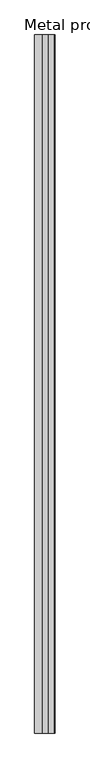
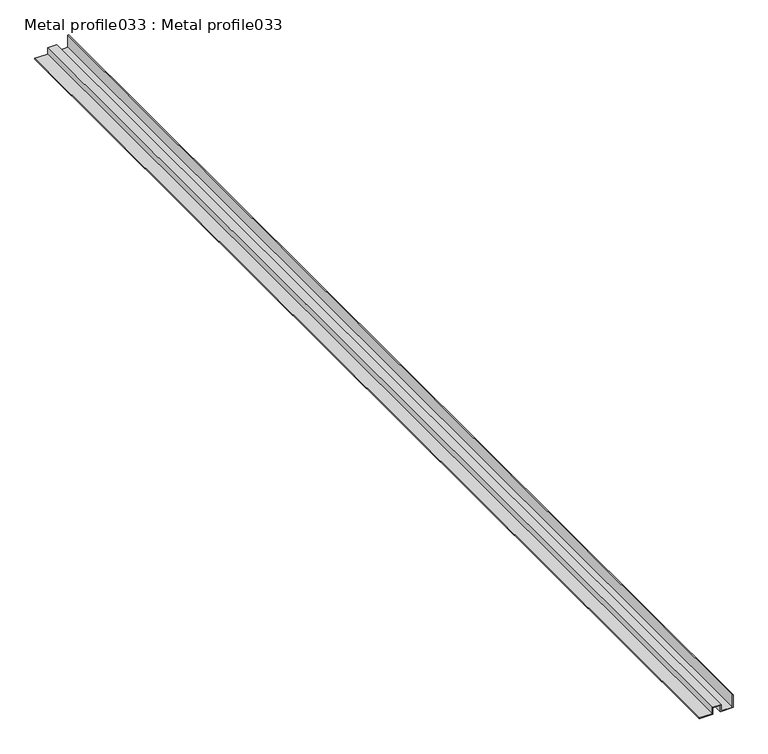
"""IFC4 building model written with IfcOpenShell, lengths in millimetres: proxy geometry, Metal profile033 : Metal profile033."""

from ifc_helpers import new_model, si_unit, frame, origin, place, context, project, spatial, polyline, outline, extrude, source, transform, mapped, element, save


def metal_profile033_metal_profile033_a58ec027(model_context):
    return source(origin(), model_context, "Body", "SweptSolid", [
        extrude(outline(polyline([(39543.8875708, -9269.4987353), (39567.6883323, -9269.4987353), (39567.6883323, -9270.7787353), (39545.1675708, -9270.7787353), (39545.1675708, -9290.4437353), (39556.5975708, -9290.4437353), (39556.5975708, -9305.7037353), (39545.1675708, -9305.7037353), (39545.1675708, -9328.1369192), (39543.8875708, -9328.1369192), (39543.8875708, -9304.4237353), (39555.3175708, -9304.4237353), (39555.3175708, -9291.7237353), (39543.8875708, -9291.7237353), (39543.8875708, -9269.4987353)])), frame((0.0, 7982.1531721, 0.0), z_axis=(0.0, 1.0, 0.0), x_axis=(0.0, 0.0, 1.0)), (0.0, 0.0, 1.0), 2000.0),
    ])


if __name__ == "__main__":
    model = new_model("IFC4")
    model_context = context("Model", 3, world=origin())
    ifc_project = project(units=[si_unit("LENGTHUNIT", "METRE", prefix="MILLI")], contexts=[model_context])
    site = spatial("IfcSite", under=ifc_project)
    building = spatial("IfcBuilding", under=site)
    placement = place(None, origin())
    metal_profile033_metal_profile033_shape = metal_profile033_metal_profile033_a58ec027(model_context)
    element("IfcBuildingElementProxy", 1, Name="Metal profile033 : Metal profile033", ObjectType="Metal profile033 : Metal profile033", at=placement, inside=building, context=model_context, shape_type="MappedRepresentation", body=[
        mapped(metal_profile033_metal_profile033_shape, transform((0.0, 0.0, 0.0), x_axis=(1.0, 0.0, 0.0), y_axis=(0.0, 1.0, 0.0), z_axis=(0.0, 0.0, 1.0))),
    ])
    save(model, "model.ifc")

# Revit data of these elements
# Type "Metal profile033 : Metal profile033"
#   NameOverride = "Metal profile033"
# Element 1 (IfcBuildingElementProxy, "Metal profile033 : Metal profile033")
#   Materials on its faces: "16 GA. COPPER SOFFIT DRIP SCREED"
# Materials
#   "16 GA. COPPER SOFFIT DRIP SCREED": class "Unassigned", colour RGB 255 217 0, transparency 0
